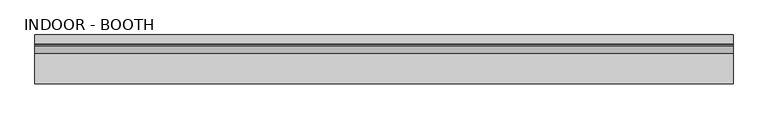
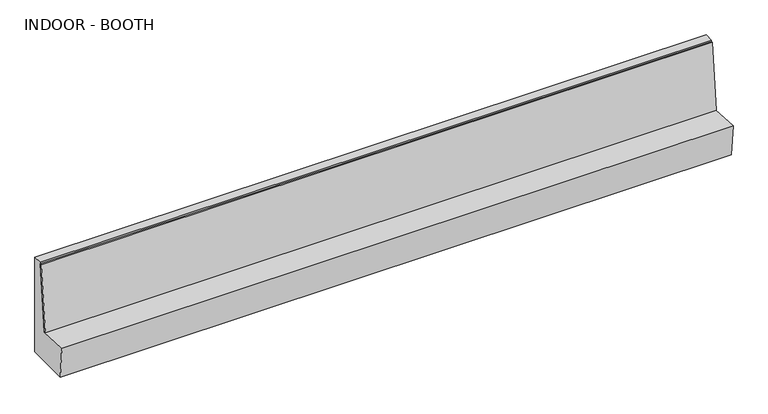
"""IFC4 building model written with IfcOpenShell, lengths in millimetres: furniture geometry, OD_CW_Booth : INDOOR - BOOTH."""

from ifc_helpers import new_model, si_unit, frame, origin, place, context, project, spatial, polyline, outline, extrude, source, transform, mapped, element, save


def indoor_booth_53f0a2fe(model_context):
    return source(origin(), model_context, "Body", "SweptSolid", [
        extrude(outline(polyline([(0.0, 9357.0837874), (25.4, 9357.0837874), (25.4, 0.0), (0.0, 0.0), (0.0, 9357.0837874)])), frame((9375.8214923, 358.2049359, 438.8309433), z_axis=(0.0, 0.10452846326765197, 0.9945218953682735), x_axis=(0.0, 0.9945218953682735, -0.10452846326765197)), (0.0, 0.0, 1.0), 944.7333479),
        extrude(outline(polyline([(609.6, 1397.0), (609.6, 0.0), (-3.4100193, 0.0), (-43.0849153, 453.4861359), (382.9385128, 431.1591941), (484.4524721, 1397.0), (609.6, 1397.0)])), frame((18.7377049, 0.0, 0.0), z_axis=(1.0, 0.0, 0.0), x_axis=(0.0, 1.0, 0.0)), (0.0, 0.0, 1.0), 9357.0837874),
    ])


if __name__ == "__main__":
    model = new_model("IFC4")
    model_context = context("Model", 3, world=origin())
    ifc_project = project(units=[si_unit("LENGTHUNIT", "METRE", prefix="MILLI")], contexts=[model_context])
    site = spatial("IfcSite", under=ifc_project)
    building = spatial("IfcBuilding", under=site)
    placement = place(None, origin())
    indoor_booth_shape = indoor_booth_53f0a2fe(model_context)
    element("IfcFurniture", 1, ObjectType="OD_CW_Booth : INDOOR - BOOTH", at=placement, inside=building, context=model_context, shape_type="MappedRepresentation", body=[
        mapped(indoor_booth_shape, transform((0.0, 0.0, 0.0), x_axis=(1.0, 0.0, 0.0), y_axis=(0.0, 1.0, 0.0), z_axis=(0.0, 0.0, 1.0))),
    ])
    save(model, "model.ifc")

# Revit data of these elements
# Type "OD_CW_Booth : INDOOR - BOOTH"
#   Type Mark = "TYPE - INDOOR - BOOTH"
#   Width = 4' - 0"
#   OD_CW_Width [instance default] = 2' - 10"
#   OD_CW_Length [instance default] = 26' - 1 83/256"
#   OD_CW_Height [instance default] = 2' - 3"
#   Height = 3' - 0"
#   Depth = 2' - 0"
#   Seating Count [instance default] = 10
#   Seating Count [instance default] = 10
#   back = Casework-oakfire
#   OD_CW_Material_Front Panel [instance default] = none
#   OD_CW_Material_Body [instance default] = none
# Element 1 (IfcFurniture, "OD_CW_Booth : INDOOR - BOOTH")
#   OD_CW_Length = 30' - 8.38913"
#   Seating Count = 11
#   OD_CW_Material_Body = WOOD-OAKFIRE
#   Materials on its faces: "WOOD-OAKFIRE", "Casework-oakfire"
# Materials
#   "Casework-oakfire": class "Miscellaneous", colour RGB 164 164 164, transparency 0, Cost = 0
#   "WOOD-OAKFIRE": class "Wood", colour RGB 198 202 183, transparency 0, Description = "Generic wood", Cost = 0
